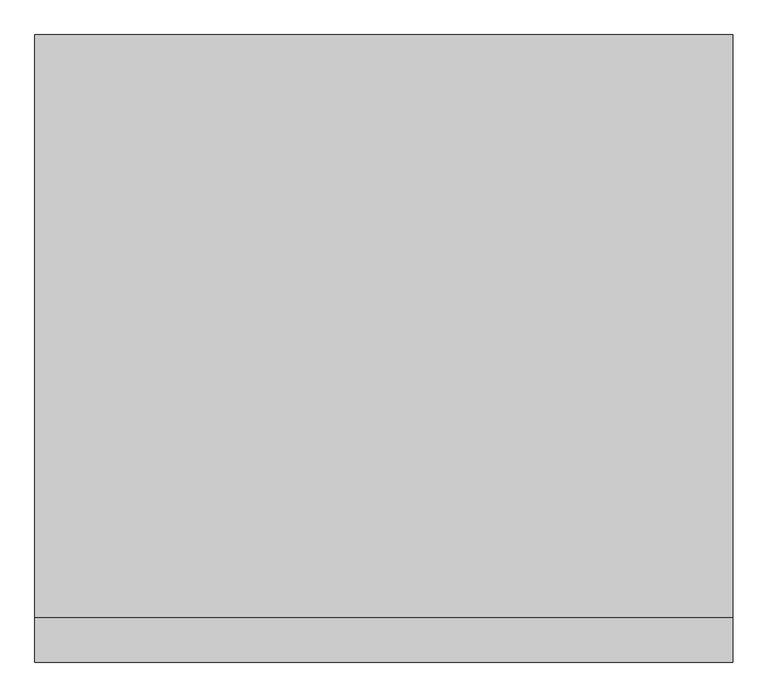
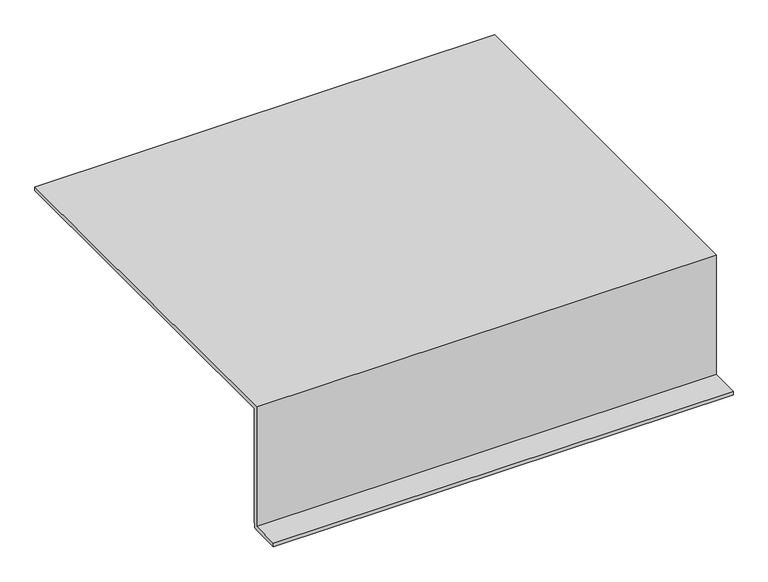
"""IFC4 building model written with IfcOpenShell, lengths in millimetres: proxy geometry, Gypsum020 34825 : Gypsum020 34825."""

import ifcopenshell
import ifcopenshell.guid

model = None  # the IFC model being written
_history = None  # IfcOwnerHistory: only IFC2X3 demands one
_inside = {}  # id of a spatial element -> (the spatial element, [elements in it])
_under = {}  # id of a project, library or spatial element -> (it, [spatial elements below it])
_declared = {}  # id of a project -> (the project, [libraries it declares])
_typed = {}  # id of a type object -> (the type object, [elements of that type])
_made_of = {}  # id of a material, layer set ... -> (it, [elements and type objects made of it])


def new_model(schema):
    """Start an empty IFC model of exactly this schema.

    Asked for "IFC4X3", IfcOpenShell would pick the latest addendum, in which some entities
    have other attributes; the version numbers below select the first issue.
    IFC2X3 requires an IfcOwnerHistory on every rooted entity: one is made here for all.
    """
    global model, _history
    if schema == "IFC4X3":
        model = ifcopenshell.file(schema_version=(4, 3, 0, 0))
    else:
        model = ifcopenshell.file(schema=schema)
    _inside.clear()
    _under.clear()
    _declared.clear()
    _typed.clear()
    _made_of.clear()
    _history = None
    if model.schema == "IFC2X3":
        org = make("IfcOrganization", Name="unknown")
        user = make(
            "IfcPersonAndOrganization",
            ThePerson=make("IfcPerson", FamilyName="unknown"),
            TheOrganization=org,
        )
        app = make(
            "IfcApplication",
            ApplicationDeveloper=org,
            Version="unknown",
            ApplicationFullName="unknown",
            ApplicationIdentifier="unknown",
        )
        _history = make(
            "IfcOwnerHistory",
            OwningUser=user,
            OwningApplication=app,
            ChangeAction="ADDED",
            CreationDate=0,
        )
    return model


def make(cls, **values):
    """One entity of the class cls with the attributes given. An attribute that is None is left unset."""
    return model.create_entity(
        cls, **{name: value for name, value in values.items() if value is not None}
    )


def rooted(cls, **values):
    """An entity with a GlobalId (a new one), such as an element, a storey or a relation."""
    return make(cls, GlobalId=ifcopenshell.guid.new(), OwnerHistory=_history, **values)


def si_unit(unit_type, name, prefix=None):
    """IfcSIUnit, for example si_unit("LENGTHUNIT", "METRE", prefix="MILLI")."""
    return make("IfcSIUnit", UnitType=unit_type, Prefix=prefix, Name=name)


def assignment(units):
    """IfcUnitAssignment: the units of a project."""
    return None if units is None else make("IfcUnitAssignment", Units=units)


def point(xyz):
    """IfcCartesianPoint."""
    return None if xyz is None else make("IfcCartesianPoint", Coordinates=xyz)


def direction(xyz):
    """IfcDirection."""
    return None if xyz is None else make("IfcDirection", DirectionRatios=xyz)


def frame(location, z_axis=None, x_axis=None):
    """IfcAxis2Placement3D, a coordinate frame: its origin and axes. An axis left out is left unset."""
    return make(
        "IfcAxis2Placement3D",
        Location=point(location),
        Axis=direction(z_axis),
        RefDirection=direction(x_axis),
    )


def origin():
    """The frame at (0, 0, 0) with its axes left unset."""
    return frame((0.0, 0.0, 0.0))


def place(relative_to, where):
    """IfcLocalPlacement: puts the frame where relative to a parent placement (None: the world)."""
    return make(
        "IfcLocalPlacement", PlacementRelTo=relative_to, RelativePlacement=where
    )


def context(
    kind, dimensions, precision=None, world=None, true_north=None, identifier=None
):
    """IfcGeometricRepresentationContext, for example the 3D "Model" context."""
    return make(
        "IfcGeometricRepresentationContext",
        ContextIdentifier=identifier,
        ContextType=kind,
        CoordinateSpaceDimension=dimensions,
        Precision=precision,
        WorldCoordinateSystem=world,
        TrueNorth=true_north,
    )


def project(units=None, contexts=None):
    """IfcProject with its units and contexts."""
    return rooted(
        "IfcProject",
        Name="project",
        RepresentationContexts=contexts,
        UnitsInContext=assignment(units),
    )


def spatial(cls, under=None, at=None, **own):
    """A site, building, storey or space (cls), placed at a placement, below another one or the project."""
    s = rooted(cls, ObjectPlacement=at, **own)
    if under is not None:
        _under.setdefault(under.id(), (under, []))[1].append(s)
    return s


def polyline(points):
    """IfcPolyline through the points."""
    return make("IfcPolyline", Points=[point(p) for p in points])


def outline(outer, holes=None, kind="AREA"):
    """IfcArbitraryClosedProfileDef: a profile drawn as a closed curve; with holes, ...WithVoids."""
    if holes is None:
        return make("IfcArbitraryClosedProfileDef", ProfileType=kind, OuterCurve=outer)
    return make(
        "IfcArbitraryProfileDefWithVoids",
        ProfileType=kind,
        OuterCurve=outer,
        InnerCurves=holes,
    )


def extrude(swept, where, along, depth):
    """IfcExtrudedAreaSolid: the profile swept, set in the frame where, extruded along a direction by depth."""
    return make(
        "IfcExtrudedAreaSolid",
        SweptArea=swept,
        Position=where,
        ExtrudedDirection=direction(along),
        Depth=depth,
    )


def shape(context_of_items, identifier, shape_type, items):
    """IfcShapeRepresentation: the items that make up one representation, for example the "Body"."""
    return make(
        "IfcShapeRepresentation",
        ContextOfItems=context_of_items,
        RepresentationIdentifier=identifier,
        RepresentationType=shape_type,
        Items=items,
    )


def source(mapping_origin, context_of_items, identifier, shape_type, items):
    """IfcRepresentationMap: a shape defined once, which mapped items show again and again."""
    return make(
        "IfcRepresentationMap",
        MappingOrigin=mapping_origin,
        MappedRepresentation=shape(context_of_items, identifier, shape_type, items),
    )


def transform(
    local_origin,
    x_axis=None,
    y_axis=None,
    z_axis=None,
    scale=None,
    scale2=None,
    scale3=None,
    uniform=True,
):
    """IfcCartesianTransformationOperator3D, or its non-uniform kind. x_axis, y_axis, z_axis: its Axis1, 2, 3."""
    if uniform:
        return make(
            "IfcCartesianTransformationOperator3D",
            Axis1=direction(x_axis),
            Axis2=direction(y_axis),
            LocalOrigin=point(local_origin),
            Scale=scale,
            Axis3=direction(z_axis),
        )
    return make(
        "IfcCartesianTransformationOperator3DnonUniform",
        Axis1=direction(x_axis),
        Axis2=direction(y_axis),
        LocalOrigin=point(local_origin),
        Scale=scale,
        Axis3=direction(z_axis),
        Scale2=scale2,
        Scale3=scale3,
    )


def mapped(mapping_source, mapping_target):
    """IfcMappedItem: shows the shape of a source again, moved by a transform."""
    return make(
        "IfcMappedItem", MappingSource=mapping_source, MappingTarget=mapping_target
    )


def made_of(thing, what):
    """Note that an element or type object is made of a material, layer set ...; save() writes the relation."""
    if what is not None:
        _made_of.setdefault(what.id(), (what, []))[1].append(thing)
    return thing


def element(
    cls,
    number,
    at=None,
    inside=None,
    cuts=None,
    type_object=None,
    material=None,
    context=None,
    identifier="Body",
    shape_type=None,
    held_by="IfcProductDefinitionShape",
    body=None,
    shapes=None,
    **own,
):
    """One element of the class cls, such as IfcWall. Its Tag is "e" and its number.

    at: its placement. inside: the storey or other place that contains it. cuts: it is an
    opening in that element (IfcRelVoidsElement). A single representation is given by context,
    identifier, shape_type and body (its items); several are given by shapes. held_by: the class
    of the entity that holds the representations. save() writes the other relations.
    """
    e = rooted(cls, Tag="e%d" % number, ObjectPlacement=at, **own)
    if body is not None:
        shapes = [shape(context, identifier, shape_type, body)]
    if shapes is not None:
        e.Representation = make(held_by, Representations=shapes)
    if inside is not None:
        _inside.setdefault(inside.id(), (inside, []))[1].append(e)
    if cuts is not None:
        rooted(
            "IfcRelVoidsElement", RelatingBuildingElement=cuts, RelatedOpeningElement=e
        )
    if type_object is not None:
        _typed.setdefault(type_object.id(), (type_object, []))[1].append(e)
    return made_of(e, material)


def aggregate(whole, parts):
    """IfcRelAggregates: a whole, such as a stair, and the parts it consists of."""
    return rooted("IfcRelAggregates", RelatingObject=whole, RelatedObjects=parts)


def save(model, path):
    """Write the relations noted so far, then the file.

    IfcRelAggregates (storeys below a building ...), IfcRelContainedInSpatialStructure (elements
    in a storey), IfcRelDefinesByType, IfcRelAssociatesMaterial and IfcRelDeclares: one each for
    every whole, place, type object, material and project.
    """
    for whole, parts in _under.values():
        aggregate(whole, parts)
    for where, things in _inside.values():
        rooted(
            "IfcRelContainedInSpatialStructure",
            RelatedElements=things,
            RelatingStructure=where,
        )
    for kind, things in _typed.values():
        rooted("IfcRelDefinesByType", RelatedObjects=things, RelatingType=kind)
    for what, things in _made_of.values():
        rooted("IfcRelAssociatesMaterial", RelatedObjects=things, RelatingMaterial=what)
    for by, libraries in _declared.values():
        rooted("IfcRelDeclares", RelatingContext=by, RelatedDefinitions=libraries)
    model.write(path)


def generic_models_33ea2bcf(model_context):
    return source(origin(), model_context, "Body", "SweptSolid", [
        extrude(outline(polyline([(-2827.7925368, 39553.8960938), (-4481.9675368, 39553.8960938), (-4481.9675368, 39025.6541813), (-4483.2475368, 39025.6541813), (-4483.2475368, 39004.5009974), (-4504.4007207, 39004.5009974), (-4504.4007207, 39003.2209974), (-4625.5194659, 39003.2209974), (-4625.5194659, 39019.0959974), (-4497.8424805, 39019.0959974), (-4497.8424805, 39569.7710938), (-2827.7925368, 39569.7710938), (-2827.7925368, 39553.8960938)])), frame((12383.0178845, 0.0, 0.0), z_axis=(1.0, 0.0, 0.0), x_axis=(0.0, 1.0, 0.0)), (0.0, 0.0, 1.0), 2000.0),
    ])


if __name__ == "__main__":
    model = new_model("IFC4")
    model_context = context("Model", 3, world=origin())
    ifc_project = project(units=[si_unit("LENGTHUNIT", "METRE", prefix="MILLI")], contexts=[model_context])
    site = spatial("IfcSite", under=ifc_project)
    building = spatial("IfcBuilding", under=site)
    placement = place(None, origin())
    generic_models_shape = generic_models_33ea2bcf(model_context)
    element("IfcBuildingElementProxy", 1, Name="Gypsum020 34825 : Gypsum020 34825", ObjectType="Gypsum020 34825 : Gypsum020 34825", at=placement, inside=building, context=model_context, shape_type="MappedRepresentation", body=[
        mapped(generic_models_shape, transform((0.0, 0.0, 0.0), x_axis=(1.0, 0.0, 0.0), y_axis=(0.0, 1.0, 0.0), z_axis=(0.0, 0.0, 1.0))),
    ])
    save(model, "model.ifc")

# Revit data of these elements
# Type "Gypsum020 34825 : Gypsum020 34825"
#   NameOverride = "Gypsum020"
# Element 1 (IfcBuildingElementProxy, "Gypsum020 34825 : Gypsum020 34825")
#   Materials on its faces: "5/8\"  GYPSUM BOARD"
# Materials
#   "5/8\"  GYPSUM BOARD": class "Unassigned", colour RGB 255 255 255, transparency 0, Cost = 0
